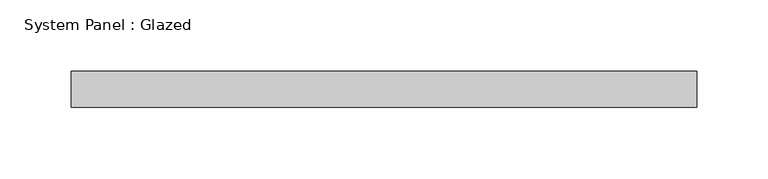
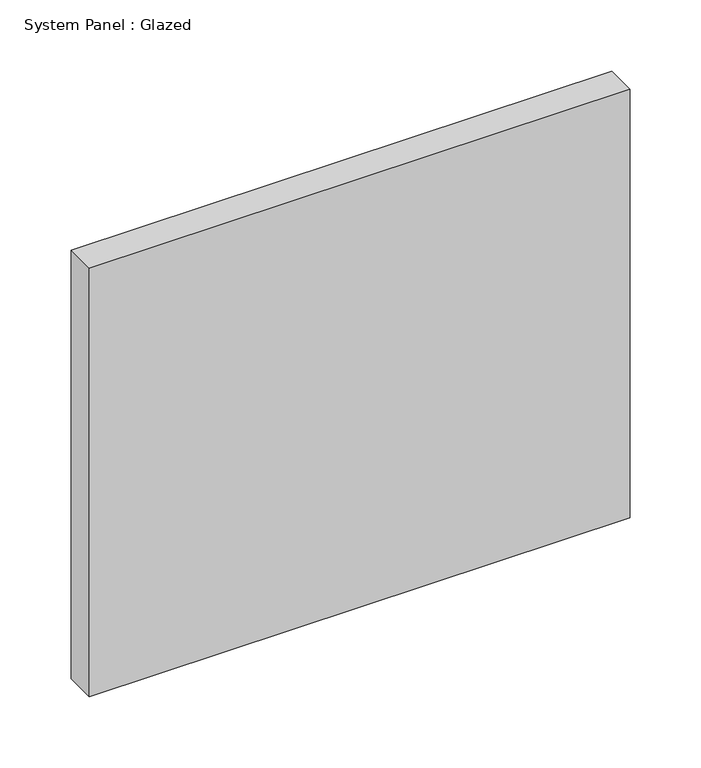
"""IFC4 building model written with IfcOpenShell, lengths in millimetres: plate geometry, System Panel : Glazed."""

from ifc_helpers import new_model, si_unit, origin, origin_with_axes, place, context, project, spatial, polyline, outline, extrude, source, transform, mapped, element, save


def system_panel_glazed_85a27524(model_context):
    return source(origin(), model_context, "Body", "SweptSolid", [
        extrude(outline(polyline([(218.9393939, 24.5), (-218.9393939, 24.5), (-218.9393939, 49.5), (218.9393939, 49.5), (218.9393939, 24.5)])), origin_with_axes(), (0.0, 0.0, 1.0), 366.6666667),
    ])


if __name__ == "__main__":
    model = new_model("IFC4")
    model_context = context("Model", 3, world=origin())
    ifc_project = project(units=[si_unit("LENGTHUNIT", "METRE", prefix="MILLI")], contexts=[model_context])
    site = spatial("IfcSite", under=ifc_project)
    building = spatial("IfcBuilding", under=site)
    placement = place(None, origin())
    system_panel_glazed_shape = system_panel_glazed_85a27524(model_context)
    element("IfcPlate", 1, ObjectType="System Panel : Glazed", at=placement, inside=building, context=model_context, shape_type="MappedRepresentation", body=[
        mapped(system_panel_glazed_shape, transform((0.0, 0.0, 0.0), x_axis=(1.0, 0.0, 0.0), y_axis=(0.0, 1.0, 0.0), z_axis=(0.0, 0.0, 1.0))),
    ])
    save(model, "model.ifc")

# Revit data of these elements
# Element 1 (IfcPlate, "System Panel : Glazed")
#   Materials on its faces: "Glass"
# Materials
#   "Glass": class "Glass", colour RGB 218 227 224, transparency 0.85, Description = "Soda Lime Glass", Cost = 0
